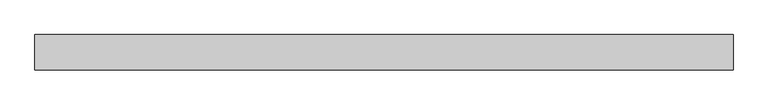
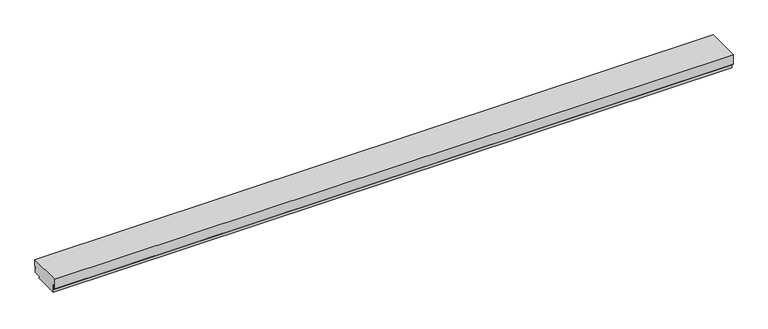
"""IFC4 building model written with IfcOpenShell, lengths in millimetres: proxy geometry, Generic Models 7:Generic Models 1:2:Generic Models 1:2 : Generic Models 7:Generic Models 1:337419:10 : Generic Models 7:Generic Models 1:2:Generic Models 1:2 : Generic Models 7:Generic Models 1:337419:306751."""

from ifc_helpers import new_model, si_unit, frame, origin, place, context, project, spatial, polyline, outline, extrude, source, transform, mapped, element, save


def generic_models_3a314b23(model_context):
    return source(origin(), model_context, "Body", "SweptSolid", [
        extrude(outline(polyline([(-536548.9570091, 2484.834375), (-536548.9570091, 2442.765625), (-536598.1695091, 2442.765625), (-536598.1695091, 2426.890625), (-536775.1757591, 2426.890625), (-536775.1757591, 2484.834375), (-536765.2538841, 2484.834375), (-536765.2538841, 2490.7875), (-536781.1288841, 2490.7875), (-536781.1288841, 2453.293898), (-536794.2257591, 2464.2834809), (-536794.2257591, 2538.4148894), (-536546.1788841, 2538.4148894), (-536546.1788841, 2490.7875), (-536558.8788841, 2490.7875), (-536558.8788841, 2484.834375), (-536548.9570091, 2484.834375)])), frame((597433.7867239, 0.0, 0.0), z_axis=(1.0, 0.0, 0.0), x_axis=(0.0, 1.0, 0.0)), (0.0, 0.0, 1.0), 4876.8),
    ])


if __name__ == "__main__":
    model = new_model("IFC4")
    model_context = context("Model", 3, world=origin())
    ifc_project = project(units=[si_unit("LENGTHUNIT", "METRE", prefix="MILLI")], contexts=[model_context])
    site = spatial("IfcSite", under=ifc_project)
    building = spatial("IfcBuilding", under=site)
    placement = place(None, origin())
    generic_models_shape = generic_models_3a314b23(model_context)
    element("IfcBuildingElementProxy", 1, Name="Generic Models 7:Generic Models 1:2:Generic Models 1:2 : Generic Models 7:Generic Models 1:337419:10 : Generic Models 7:Generic Models 1:2:Generic Models 1:2 : Generic Models 7:Generic Models 1:337419:306751", ObjectType="Generic Models 7:Generic Models 1:2:Generic Models 1:2 : Generic Models 7:Generic Models 1:337419:10 : Generic Models 7:Generic Models 1:2:Generic Models 1:2 : Generic Models 7:Generic Models 1:337419:306751", at=placement, inside=building, context=model_context, shape_type="MappedRepresentation", body=[
        mapped(generic_models_shape, transform((0.0, 0.0, 0.0), x_axis=(1.0, 0.0, 0.0), y_axis=(0.0, 1.0, 0.0), z_axis=(0.0, 0.0, 1.0))),
    ])
    save(model, "model.ifc")

# Revit data of these elements
# Type "Generic Models 7:Generic Models 1:2:Generic Models 1:2 : Generic Models 7:Generic Models 1:337419:10 : Generic Models 7:Generic Models 1:2:Generic Models 1:2 : Generic Models 7:Generic Models 1:337419:306751"
#   NameOverride = "Generic Models 7:Generic Models 1:2:Generic Models 1:2 : Generic Models 7:Generic Models 1:337419:306751"
#   ObjectTypeOverride = "Generic Models 1:2 : Generic Models 7:Generic Models 1:337419"
#   Reference = "Generic Models 1"
#   Tag = "306751"
# Element 1 (IfcBuildingElementProxy, "Generic Models 7:Generic Models 1:2:Generic Models 1:2 : Generic Models 7:Generic Models 1:337419:10 : Generic Models 7:Generic Models 1:2:Generic Models 1:2 : Generic Models 7:Generic Models 1:337419:306751")
#   Materials on its faces: "LOW VOLUMN EXPANDABLE FOAM INSULATION"
# Materials
#   "LOW VOLUMN EXPANDABLE FOAM INSULATION": class "Unassigned", colour RGB 213 216 95, transparency 0, Cost = 0
